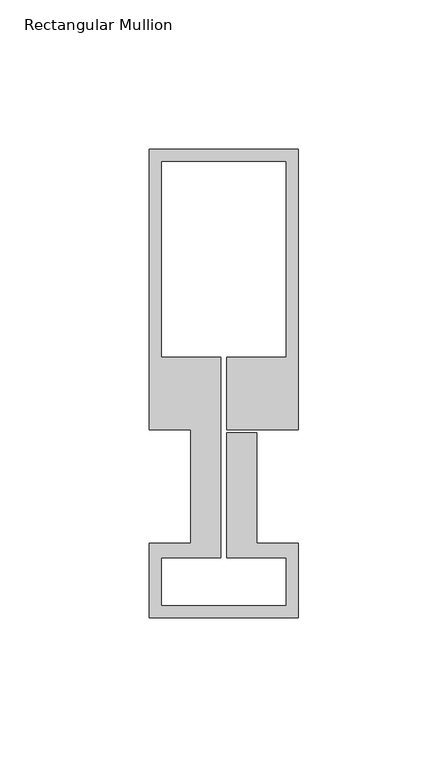
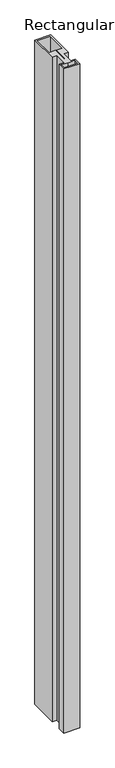
"""IFC4 building model written with IfcOpenShell, lengths in millimetres: member geometry, Rectangular Mullion : Schueco_FWS-50-SI_Mull_CovCap-20mm_Mull-85mm."""

from ifc_helpers import new_model, si_unit, frame, origin, place, context, project, spatial, polyline, outline, extrude, source, transform, mapped, element, save


def rectangular_mullion_9473cae2(model_context):
    return source(origin(), model_context, "Body", "SweptSolid", [
        extrude(outline(polyline([(-50.0, 132.0), (0.0, 132.0), (0.0, 38.0), (-24.0, 38.0), (-24.0, 62.3), (-4.0, 62.3), (-4.0, 128.0), (-46.0, 128.0), (-46.0, 62.3), (-26.0, 62.3), (-26.0, -5.0), (-46.0, -5.0), (-46.0, -21.0), (-4.0, -21.0), (-4.0, -5.0), (-24.0, -5.0), (-24.0, 37.0), (-14.0, 37.0), (-14.0, -0.1), (0.0, -0.1), (0.0, -25.0), (-50.0, -25.0), (-50.0, -0.1), (-36.0, -0.1), (-36.0, 38.0), (-50.0, 38.0), (-50.0, 132.0)])), frame((0.0, 0.0, -2200.0), z_axis=(0.0, 0.0, 1.0), x_axis=(1.0, 0.0, 0.0)), (0.0, 0.0, 1.0), 2200.0),
    ])


if __name__ == "__main__":
    model = new_model("IFC4")
    model_context = context("Model", 3, world=origin())
    ifc_project = project(units=[si_unit("LENGTHUNIT", "METRE", prefix="MILLI")], contexts=[model_context])
    site = spatial("IfcSite", under=ifc_project)
    building = spatial("IfcBuilding", under=site)
    placement = place(None, origin())
    rectangular_mullion_shape = rectangular_mullion_9473cae2(model_context)
    element("IfcMember", 1, ObjectType="Rectangular Mullion : Schueco_FWS-50-SI_Mull_CovCap-20mm_Mull-85mm", at=placement, inside=building, context=model_context, shape_type="MappedRepresentation", body=[
        mapped(rectangular_mullion_shape, transform((0.0, 0.0, 0.0), x_axis=(1.0, 0.0, 0.0), y_axis=(0.0, 1.0, 0.0), z_axis=(0.0, 0.0, 1.0))),
    ])
    save(model, "model.ifc")

# Revit data of these elements
# Type "Rectangular Mullion : Schueco_FWS-50-SI_Mull_CovCap-20mm_Mull-85mm"
#   Model = "FWS 50.SI"
#   Manufacturer = "Schueco International KG"
#   Type Comments = "Mullion"
#   Schueco thermal insulation standard = "Suitable for passive houses"
#   Burglar resistance = "RC 3"
#   Thermal insulation = "to 0.70 W/(m²K)"
#   built-in parameter 1007322 = 0.515092 (stored number, unit not read)
#   built-in parameter 1007321 = 0.0360892 (stored number, unit not read)
#   built-in parameter 1007320 = 0.0360892 (stored number, unit not read)
# Element 1 (IfcMember, "Rectangular Mullion : Schueco_FWS-50-SI_Mull_CovCap-20mm_Mull-85mm")
#   Materials on its faces: "Alu"
# Materials
#   "Alu": class "Glas", colour RGB 140 140 140, transparency 0
